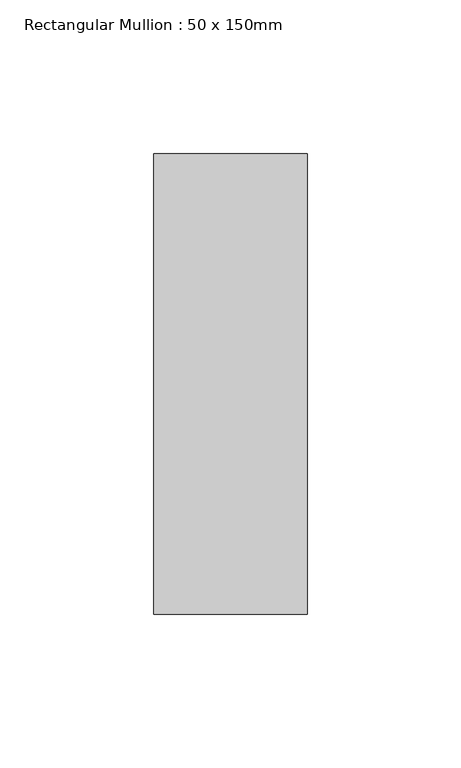
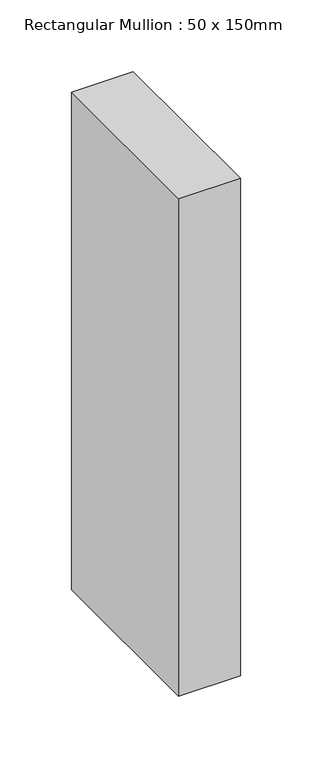
"""IFC4 building model written with IfcOpenShell, lengths in millimetres: member geometry, Rectangular Mullion : 50 x 150mm."""

from ifc_helpers import new_model, si_unit, frame, origin, place, context, project, spatial, polyline, outline, extrude, source, transform, mapped, element, save


def rectangular_mullion_50_x_150mm_8076e6a0(model_context):
    return source(origin(), model_context, "Body", "SweptSolid", [
        extrude(outline(polyline([(0.0, 75.0), (0.0, -75.0), (-50.0, -75.0), (-50.0, 75.0), (0.0, 75.0)])), frame((0.0, 0.0, -425.0000001), z_axis=(0.0, 0.0, 1.0), x_axis=(1.0, 0.0, 0.0)), (0.0, 0.0, 1.0), 425.0000001),
    ])


if __name__ == "__main__":
    model = new_model("IFC4")
    model_context = context("Model", 3, world=origin())
    ifc_project = project(units=[si_unit("LENGTHUNIT", "METRE", prefix="MILLI")], contexts=[model_context])
    site = spatial("IfcSite", under=ifc_project)
    building = spatial("IfcBuilding", under=site)
    placement = place(None, origin())
    rectangular_mullion_50_x_150mm_shape = rectangular_mullion_50_x_150mm_8076e6a0(model_context)
    element("IfcMember", 1, ObjectType="Rectangular Mullion : 50 x 150mm", at=placement, inside=building, context=model_context, shape_type="MappedRepresentation", body=[
        mapped(rectangular_mullion_50_x_150mm_shape, transform((0.0, 0.0, 0.0), x_axis=(1.0, 0.0, 0.0), y_axis=(0.0, 1.0, 0.0), z_axis=(0.0, 0.0, 1.0))),
    ])
    save(model, "model.ifc")

# Revit data of these elements
# Type "Rectangular Mullion : 50 x 150mm"
#   built-in parameter 1007304 = 0.492126 (stored number, unit not read)
#   built-in parameter 1007301 = 0.082021 (stored number, unit not read)
#   built-in parameter 1007300 = 0.082021 (stored number, unit not read)
# Element 1 (IfcMember, "Rectangular Mullion : 50 x 150mm")
#   Materials on its faces: "Aluminium"
# Materials
#   "Aluminium": class "Metal", colour RGB 247 247 247, transparency 0, Description = "Aluminium 6061", Cost = 0
